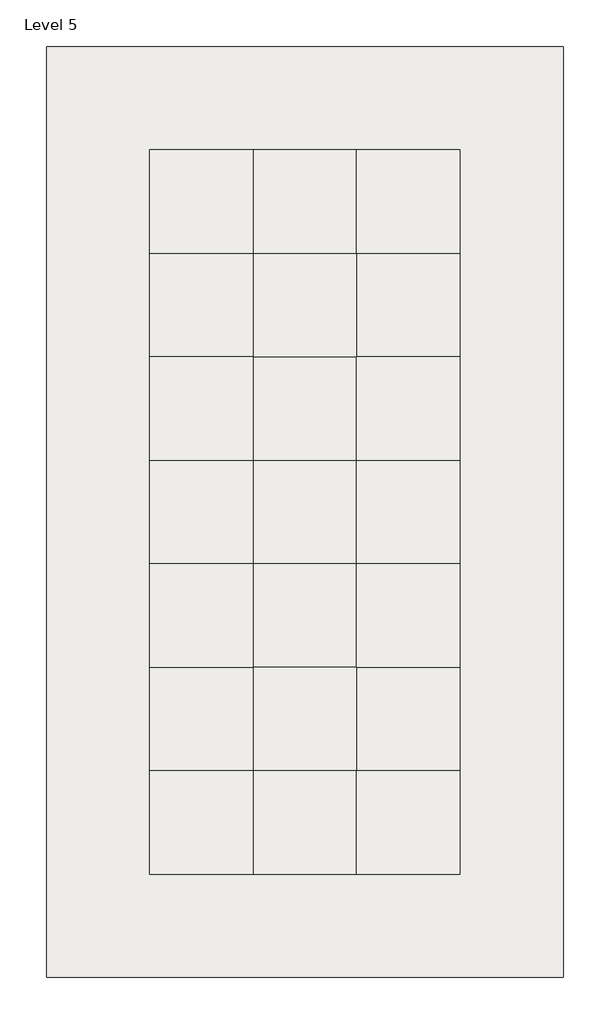
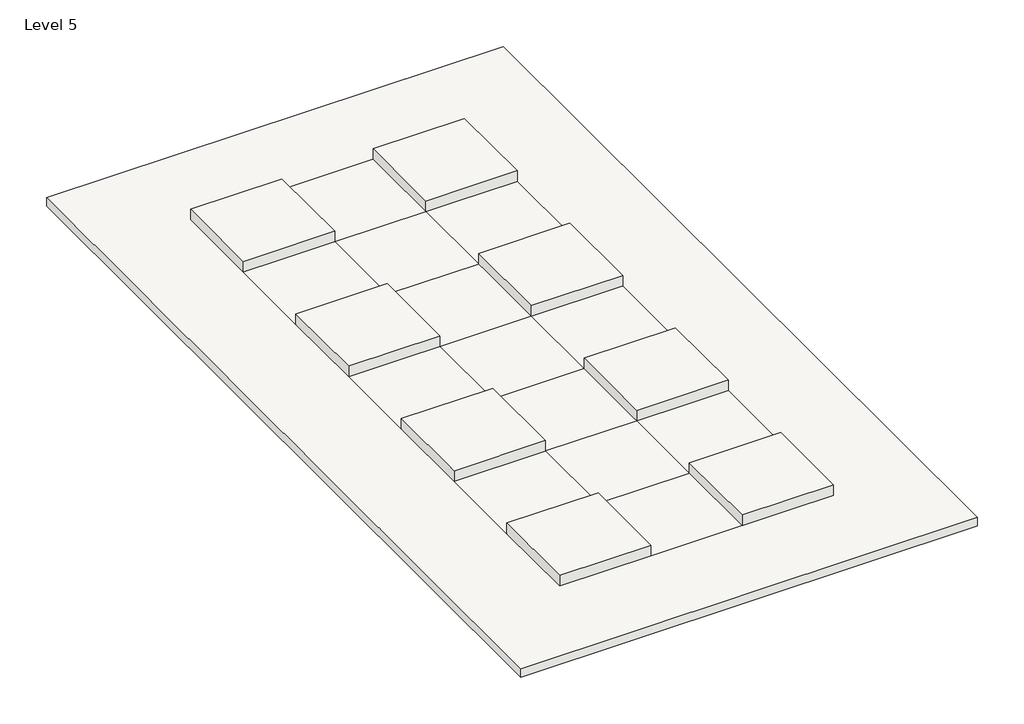
# One storey: 9 roofs.
"""IFC4 building model written with IfcOpenShell, lengths in millimetres."""

from ifc_helpers import new_model, si_unit, origin, place, context, project, spatial, faceted_brep, element, save

model = new_model("IFC4")

# Units and contexts
model_context = context("Model", 3, world=origin())
ifc_project = project(units=[si_unit("LENGTHUNIT", "METRE", prefix="MILLI")], contexts=[model_context])

# Site, building, storey
site = spatial("IfcSite", under=ifc_project)
building = spatial("IfcBuilding", under=site)
storey = spatial("IfcBuildingStorey", under=building, Name="Level 5", Elevation=20000.0)

# Roofs
placement = place(None, origin())
element("IfcRoof", 1, ObjectType="Bauder_RoofCoveringSystem_ExtensiveGreenRoofSystem_WildflowerBlanket", at=placement, inside=storey, context=model_context, shape_type="Brep", body=[
    faceted_brep([(-674.7340554, 1676.2074539, 20000.0), (1325.2659446, 1676.2074539, 20000.0), (1325.2659446, -323.7925461, 20000.0), (-674.7340554, -323.7925461, 20000.0), (1325.2659446, 1676.2074539, 20445.0), (-674.7340554, 1676.2074539, 20445.0), (-674.7340554, -323.7925461, 20445.0), (1325.2659446, -323.7925461, 20445.0), (1325.2659446, 1676.2074539, 20200.0), (-674.7340554, 1676.2074539, 20200.0), (-674.7340554, -323.7925461, 20200.0), (1325.2659446, -323.7925461, 20200.0)], [[[0, 1, 2, 3]], [[4, 5, 6, 7]], [[5, 4, 8, 1, 0, 9]], [[6, 5, 9, 0, 3, 10]], [[7, 6, 10, 3, 2, 11]], [[4, 7, 11, 2, 1, 8]]]),
])
element("IfcRoof", 2, ObjectType="Bauder_RoofCoveringSystem_ExtensiveGreenRoofSystem_WildflowerBlanket", at=placement, inside=storey, context=model_context, shape_type="Brep", body=[
    faceted_brep([(3325.2659446, 1676.2074539, 20000.0), (5325.2659446, 1676.2074539, 20000.0), (5325.2659446, -323.7925461, 20000.0), (3325.2659446, -323.7925461, 20000.0), (5325.2659446, 1676.2074539, 20445.0), (3325.2659446, 1676.2074539, 20445.0), (3325.2659446, -323.7925461, 20445.0), (5325.2659446, -323.7925461, 20445.0), (5325.2659446, 1676.2074539, 20200.0), (3325.2659446, 1676.2074539, 20200.0), (3325.2659446, -323.7925461, 20200.0), (5325.2659446, -323.7925461, 20200.0)], [[[0, 1, 2, 3]], [[4, 5, 6, 7]], [[5, 4, 8, 1, 0, 9]], [[6, 5, 9, 0, 3, 10]], [[7, 6, 10, 3, 2, 11]], [[4, 7, 11, 2, 1, 8]]]),
])
element("IfcRoof", 3, ObjectType="Bauder_RoofCoveringSystem_ExtensiveGreenRoofSystem_WildflowerBlanket", at=placement, inside=storey, context=model_context, shape_type="Brep", body=[
    faceted_brep([(3325.2659446, -2323.7925461, 20000.0), (5325.2659446, -2323.7925461, 20000.0), (5325.2659446, -4323.7925461, 20000.0), (3325.2659446, -4323.7925461, 20000.0), (5325.2659446, -2323.7925461, 20445.0), (3325.2659446, -2323.7925461, 20445.0), (3325.2659446, -4323.7925461, 20445.0), (5325.2659446, -4323.7925461, 20445.0), (5325.2659446, -2323.7925461, 20200.0), (3325.2659446, -2323.7925461, 20200.0), (3325.2659446, -4323.7925461, 20200.0), (5325.2659446, -4323.7925461, 20200.0)], [[[0, 1, 2, 3]], [[4, 5, 6, 7]], [[5, 4, 8, 1, 0, 9]], [[6, 5, 9, 0, 3, 10]], [[7, 6, 10, 3, 2, 11]], [[4, 7, 11, 2, 1, 8]]]),
])
element("IfcRoof", 4, ObjectType="Bauder_RoofCoveringSystem_ExtensiveGreenRoofSystem_WildflowerBlanket", at=placement, inside=storey, context=model_context, shape_type="Brep", body=[
    faceted_brep([(3325.2659446, -6323.7925461, 20000.0), (5325.2659446, -6323.7925461, 20000.0), (5325.2659446, -8323.7925461, 20000.0), (3325.2659446, -8323.7925461, 20000.0), (5325.2659446, -6323.7925461, 20445.0), (3325.2659446, -6323.7925461, 20445.0), (3325.2659446, -8323.7925461, 20445.0), (5325.2659446, -8323.7925461, 20445.0), (3325.2659446, -6323.7925461, 20200.0), (5325.2659446, -6323.7925461, 20200.0), (3325.2659446, -8323.7925461, 20200.0), (5325.2659446, -8323.7925461, 20200.0)], [[[0, 1, 2, 3]], [[4, 5, 6, 7]], [[0, 8, 5, 4, 9, 1]], [[3, 10, 6, 5, 8, 0]], [[2, 11, 7, 6, 10, 3]], [[1, 9, 4, 7, 11, 2]]]),
])
element("IfcRoof", 5, ObjectType="Bauder_RoofCoveringSystem_ExtensiveGreenRoofSystem_WildflowerBlanket", at=placement, inside=storey, context=model_context, shape_type="Brep", body=[
    faceted_brep([(3325.2659446, -10323.7925461, 20000.0), (5325.2659446, -10323.7925461, 20000.0), (5325.2659446, -12323.7925461, 20000.0), (3325.2659446, -12323.7925461, 20000.0), (5325.2659446, -10323.7925461, 20445.0), (3325.2659446, -10323.7925461, 20445.0), (3325.2659446, -12323.7925461, 20445.0), (5325.2659446, -12323.7925461, 20445.0), (3325.2659446, -10323.7925461, 20200.0), (5325.2659446, -10323.7925461, 20200.0), (3325.2659446, -12323.7925461, 20200.0), (5325.2659446, -12323.7925461, 20200.0)], [[[0, 1, 2, 3]], [[4, 5, 6, 7]], [[0, 8, 5, 4, 9, 1]], [[3, 10, 6, 5, 8, 0]], [[2, 11, 7, 6, 10, 3]], [[1, 9, 4, 7, 11, 2]]]),
])
element("IfcRoof", 6, ObjectType="Bauder_RoofCoveringSystem_ExtensiveGreenRoofSystem_WildflowerBlanket", at=placement, inside=storey, context=model_context, shape_type="Brep", body=[
    faceted_brep([(-674.7340554, -10323.7925461, 20000.0), (1325.2659446, -10323.7925461, 20000.0), (1325.2659446, -12323.7925461, 20000.0), (-674.7340554, -12323.7925461, 20000.0), (1325.2659446, -10323.7925461, 20445.0), (-674.7340554, -10323.7925461, 20445.0), (-674.7340554, -12323.7925461, 20445.0), (1325.2659446, -12323.7925461, 20445.0), (1325.2659446, -10323.7925461, 20200.0), (-674.7340554, -10323.7925461, 20200.0), (-674.7340554, -12323.7925461, 20200.0), (1325.2659446, -12323.7925461, 20200.0)], [[[0, 1, 2, 3]], [[4, 5, 6, 7]], [[5, 4, 8, 1, 0, 9]], [[6, 5, 9, 0, 3, 10]], [[7, 6, 10, 3, 2, 11]], [[4, 7, 11, 2, 1, 8]]]),
])
element("IfcRoof", 7, ObjectType="Bauder_RoofCoveringSystem_ExtensiveGreenRoofSystem_WildflowerBlanket", at=placement, inside=storey, context=model_context, shape_type="Brep", body=[
    faceted_brep([(-674.7340554, -6323.7925461, 20000.0), (1325.2659446, -6323.7925461, 20000.0), (1325.2659446, -8323.7925461, 20000.0), (-674.7340554, -8323.7925461, 20000.0), (1325.2659446, -6323.7925461, 20445.0), (-674.7340554, -6323.7925461, 20445.0), (-674.7340554, -8323.7925461, 20445.0), (1325.2659446, -8323.7925461, 20445.0), (1325.2659446, -6323.7925461, 20200.0), (-674.7340554, -6323.7925461, 20200.0), (-674.7340554, -8323.7925461, 20200.0), (1325.2659446, -8323.7925461, 20200.0)], [[[0, 1, 2, 3]], [[4, 5, 6, 7]], [[5, 4, 8, 1, 0, 9]], [[6, 5, 9, 0, 3, 10]], [[7, 6, 10, 3, 2, 11]], [[4, 7, 11, 2, 1, 8]]]),
])
element("IfcRoof", 8, ObjectType="Bauder_RoofCoveringSystem_ExtensiveGreenRoofSystem_WildflowerBlanket", at=placement, inside=storey, context=model_context, shape_type="Brep", body=[
    faceted_brep([(-674.7340554, -2323.7925461, 20000.0), (1325.2659446, -2323.7925461, 20000.0), (1325.2659446, -4323.7925461, 20000.0), (-674.7340554, -4323.7925461, 20000.0), (1325.2659446, -2323.7925461, 20445.0), (-674.7340554, -2323.7925461, 20445.0), (-674.7340554, -4323.7925461, 20445.0), (1325.2659446, -4323.7925461, 20445.0), (1325.2659446, -2323.7925461, 20200.0), (-674.7340554, -2323.7925461, 20200.0), (-674.7340554, -4323.7925461, 20200.0), (1325.2659446, -4323.7925461, 20200.0)], [[[0, 1, 2, 3]], [[4, 5, 6, 7]], [[5, 4, 8, 1, 0, 9]], [[6, 5, 9, 0, 3, 10]], [[7, 6, 10, 3, 2, 11]], [[4, 7, 11, 2, 1, 8]]]),
])
element("IfcRoof", 9, ObjectType="Roof_Concrete-200mm", at=placement, inside=storey, context=model_context, shape_type="Brep", body=[
    faceted_brep([(-2674.7340554, -14323.7925461, 20200.0), (-2674.7340554, -14323.7925461, 20000.0), (7325.2659446, -14323.7925461, 20000.0), (7325.2659446, -14323.7925461, 20200.0), (-2674.7340554, 3676.2074539, 20200.0), (-2674.7340554, 3676.2074539, 20000.0), (7325.2659446, 3676.2074539, 20200.0), (7325.2659446, 3676.2074539, 20000.0), (3325.2659446, 1676.2074539, 20200.0), (1325.2659446, 1676.2074539, 20200.0), (1325.2659446, -323.7925461, 20200.0), (3325.2659446, -323.7925461, 20200.0), (1325.2659446, 1676.2074539, 20000.0), (3325.2659446, 1676.2074539, 20000.0), (3325.2659446, -323.7925461, 20000.0), (1325.2659446, -323.7925461, 20000.0), (1325.2659446, -2323.7925461, 20200.0), (-674.7340554, -323.7925461, 20200.0), (-674.7340554, -2323.7925461, 20200.0), (3325.2659446, -2323.7925461, 20200.0), (5325.2659446, -2323.7925461, 20200.0), (5325.2659446, -323.7925461, 20200.0), (-674.7340554, -2323.7925461, 20000.0), (-674.7340554, -323.7925461, 20000.0), (1325.2659446, -2323.7925461, 20000.0), (3325.2659446, -2323.7925461, 20000.0), (5325.2659446, -323.7925461, 20000.0), (5325.2659446, -2323.7925461, 20000.0), (1325.2659446, -4323.7925461, 20200.0), (3325.2659446, -4323.7925461, 20200.0), (3325.2659446, -4323.7925461, 20000.0), (1325.2659446, -4323.7925461, 20000.0), (1325.2659446, -6323.7925461, 20200.0), (-674.7340554, -4323.7925461, 20200.0), (-674.7340554, -6323.7925461, 20200.0), (5325.2659446, -6323.7925461, 20200.0), (5325.2659446, -4323.7925461, 20200.0), (3325.2659446, -6323.7925461, 20200.0), (-674.7340554, -6323.7925461, 20000.0), (-674.7340554, -4323.7925461, 20000.0), (1325.2659446, -6323.7925461, 20000.0), (3325.2659446, -6323.7925461, 20000.0), (5325.2659446, -4323.7925461, 20000.0), (5325.2659446, -6323.7925461, 20000.0), (1325.2659446, -12323.7925461, 20200.0), (3325.2659446, -12323.7925461, 20200.0), (3325.2659446, -10323.7925461, 20200.0), (1325.2659446, -10323.7925461, 20200.0), (3325.2659446, -12323.7925461, 20000.0), (1325.2659446, -12323.7925461, 20000.0), (1325.2659446, -10323.7925461, 20000.0), (3325.2659446, -10323.7925461, 20000.0), (1325.2659446, -8323.7925461, 20200.0), (-674.7340554, -8323.7925461, 20200.0), (-674.7340554, -10323.7925461, 20200.0), (3325.2659446, -8323.7925461, 20200.0), (5325.2659446, -10323.7925461, 20200.0), (5325.2659446, -8323.7925461, 20200.0), (-674.7340554, -10323.7925461, 20000.0), (-674.7340554, -8323.7925461, 20000.0), (1325.2659446, -8323.7925461, 20000.0), (3325.2659446, -8323.7925461, 20000.0), (5325.2659446, -8323.7925461, 20000.0), (5325.2659446, -10323.7925461, 20000.0), (-674.7340554, 1676.2074539, 20000.0), (-674.7340554, 1676.2074539, 20200.0), (5325.2659446, 1676.2074539, 20200.0), (5325.2659446, 1676.2074539, 20000.0), (5325.2659446, -12323.7925461, 20000.0), (5325.2659446, -12323.7925461, 20200.0), (-674.7340554, -12323.7925461, 20000.0), (-674.7340554, -12323.7925461, 20200.0)], [[[0, 1, 2, 3]], [[1, 0, 4, 5]], [[6, 7, 5, 4]], [[3, 2, 7, 6]], [[8, 9, 10, 11]], [[12, 13, 14, 15]], [[16, 10, 17, 18]], [[11, 10, 16, 19]], [[20, 21, 11, 19]], [[22, 23, 15, 24]], [[15, 14, 25, 24]], [[25, 14, 26, 27]], [[19, 16, 28, 29]], [[24, 25, 30, 31]], [[32, 28, 33, 34]], [[35, 36, 29, 37]], [[38, 39, 31, 40]], [[41, 30, 42, 43]], [[44, 45, 46, 47]], [[48, 49, 50, 51]], [[47, 52, 53, 54]], [[47, 46, 55, 52]], [[56, 57, 55, 46]], [[58, 59, 60, 50]], [[51, 50, 60, 61]], [[51, 61, 62, 63]], [[52, 55, 37, 32]], [[29, 28, 32, 37]], [[61, 60, 40, 41]], [[31, 30, 41, 40]], [[9, 12, 15, 10]], [[10, 15, 23, 17]], [[17, 23, 64, 65]], [[12, 9, 65, 64]], [[66, 67, 26, 21]], [[21, 26, 14, 11]], [[11, 14, 13, 8]], [[67, 66, 8, 13]], [[20, 27, 42, 36]], [[36, 42, 30, 29]], [[29, 30, 25, 19]], [[27, 20, 19, 25]], [[16, 24, 31, 28]], [[28, 31, 39, 33]], [[33, 39, 22, 18]], [[24, 16, 18, 22]], [[32, 40, 60, 52]], [[52, 60, 59, 53]], [[53, 59, 38, 34]], [[40, 32, 34, 38]], [[35, 43, 62, 57]], [[57, 62, 61, 55]], [[55, 61, 41, 37]], [[43, 35, 37, 41]], [[56, 63, 68, 69]], [[69, 68, 48, 45]], [[45, 48, 51, 46]], [[63, 56, 46, 51]], [[47, 50, 49, 44]], [[44, 49, 70, 71]], [[71, 70, 58, 54]], [[50, 47, 54, 58]], [[4, 0, 3, 6], [9, 8, 66, 21, 20, 36, 35, 57, 56, 69, 45, 44, 71, 54, 53, 34, 33, 18, 17, 65]], [[7, 2, 1, 5], [13, 12, 64, 23, 22, 39, 38, 59, 58, 70, 49, 48, 68, 63, 62, 43, 42, 27, 26, 67]]]),
])

save(model, "model.ifc")

# Revit data of these elements
# Type "Bauder_RoofCoveringSystem_ExtensiveGreenRoofSystem_WildflowerBlanket"
#   Keynote = "Q37"
#   Type IFC Predefined Type = "FLAT_ROOF"
#   Export Type to IFC As = "IfcRoofType"
#   Model = "Bauder Biodiverse Wildflower Blanket - Extensive Green Roof System"
#   Manufacturer = "Bauder Ltd"
#   Type Comments = "Wildflower Blanket"
#   URL = "https://www.bauder.co.uk/"
#   Description = "Bauder Biodiverse GreenRoof system incorporating WB 25 mm UK Native Species Wildflower Blanket with Biodiverse Substrate, Filter Fleece, DSE40 Polyethylene Drainage and Protection Layer, and FSM600 Polyester-Polypropylene fibre protection mat."
#   Assembly Code = "B3010"
#   NBSDescription = "Extensive green roof system"
#   NBSReference = "45-40-47/130"
#   BIMObjectName = "Bauder_RoofCoveringSystem_ExtensiveGreenRoofSystem_WildflowerBlanket"
#   AccessibilityPerformance = "n/a"
#   CodePerformance = "n/a"
#   Color = "n/a"
#   Constituents = "n/a"
#   DurationUnit = "Year"
#   ExpectedLife = "n/a"
#   Features = "This BIM Object must be supported by a project specific specification from Bauder, incorporating system build-up, detail design and performance calculations if a full Bauder system guarantee is required. Please contact your local Bauder Representative or technical@bauder.co.uk"
#   Finish = "n/a"
#   Grade = "n/a"
#   Material = "n/a"
#   ModelReference = "Bauder Biodiverse Wildflower Blanket - Extensive Green Roof System"
#   Name = "RoofCoveringSystem_Bauder_ExtensiveGreenRoofSystem"
#   ReplacementCost = "n/a"
#   Shape = "n/a"
#   Size = "n/a"
#   SustainabilityPerformance = "Bauder Germany ISO14001: Certificate No.: 70499/03-15 e, Bauder UK ISO14001:Certificate No. 19ACM6595R, EN1271, BREEAM Credits Available"
#   WarrantyDescription = "Guarantee options could include ‘Product’, ‘Product and Workmanship’ and ‘Product, Workmanship and Design’ Guarantees. All guarantees available for this system are subject to the works being carried out in accordance with the Bauder specification and being installed by a Bauder Approved installer. For full details and further information regarding guarantees and alternative systems please contact your local Bauder Representative or technical@bauder.co.uk"
#   WarrantyDurationLabor = "n/a"
#   WarrantyDurationParts = "n/a"
#   WarrantyDurationUnit = "Year"
#   WarrantyGuarantorLabor = "n/a"
#   WarrantyGuarantorParts = "technical@bauder.co.uk"
#   Certification = "Comply with GRO Green Roof Code of Practice and FLL Standards"
#   EdgeRestraints = "Perforated edge trim where required, refer to Bauder Project Specific Specification"
#   MoistureControlDrainageAncillaries = "n/a"
#   MoistureControlDrainageLayer = "Bauder DSE40 40 mm Polyethylene Drainage and Protection Layer"
#   MoistureControlFilterMembrane = "Bauder Filter Fleece 1 mm Polypropylene Filter Fleece"
#   MoistureControlMoistureRetentionMat = "Polypropylene mesh bonded to a moisture permeable base carrier sheet integral to the Blanket"
#   PlantingSystemsAntierosionMat = "Jute Net where exposed, refer to Bauder Project Specific Specification"
#   PlantingSystemsPlantingMedium = "Bauder Biodiverse Substrate Recycled crushed brick, expanded clay shale and composted pine bark"
#   PlantingSystemsVegetation = "Bauder WB 25 mm UK Native Species Wildflower Blanket"
#   PlantingSystemsVegetationBarrier = "20-40 mm Rounded-Washed Stones, refer to Bauder Project Specific Specification"
#   ProjectSpecificationAndDesign = "This BIM Object must be supported by a project specific specification from Bauder, incorporating system build-up, detail design and performance calculations if a full Bauder system warranty is required. Please contact your local Bauder Representative or technical@bauder.co.uk"
#   ProtectionProtectionLayer = "Bauder FSM600 4 mm Polyester-Polypropylene fibre protection mat"
#   ProtectionRootBarrier = "As per project specific Bauder Specification"
#   ProtectionSeparationLayer = "n/a"
#   SystemManufacturer = "Bauder Ltd"
#   WarrantyConsiderations = "All guarantees available for this system are subject to the works being carried out in accordance with the Bauder specification and being installed by a Bauder Approved installer. For full details and further information regarding guarantees and alternative systems please contact your local Bauder Representative or technical@bauder.co.uk"
#   Update = "1900-12-31T23:59:59"
#   Documentation = "https://www.bauder.co.uk/technical-centre/technical-literature/system-brochures"
#   DocumentReference = "http://www.bauder.co.uk/"
#   IfcExportAs = "IfcRoofType"
#   IfcExportType = "FLAT_ROOF"
#   MethodOfMesurement = "n/a"
#   Process = "Replacement at service life intervals"
#   FireRating = "n/a"
#   _Author = "AM"
#   _AuthorizedBy = "bimstore"
#   _CreatedBy = "technical@bauder.co.uk"
#   _DistributedBy = "www.bimstore.co"
#   AssetType = "Fixed"
#   ClassificationName = "Uniclass2015"
#   ClassificationValue = "Ss_45_40_47_09"
#   CreatedBy = "technical@bauder.co.uk"
#   CreatedOn = "2023-02-10 T00:00:00"
#   DocumentationCertificates = "n/a"
#   DocumentationInstallationGuide = "https://www.bauder.co.uk/technical-centre"
#   DocumentationLiterature = "https://www.bauder.co.uk/technical-centre"
#   DocumentationMaintenance = "https://www.bauder.co.uk/technical-centre/maintenance-advice"
#   DocumentationTechnical = "https://www.bauder.co.uk/green-roofs/extensive-green-roofs/biodiverse-or-brown-roofs/wildflower-blanket"
#   ManufacturerName = "Bauder Ltd"
#   ModelNumber = "0905_WB-BioS-FF-D4-F6"
#   ProductionYear = "2017"
#   ReferencedStandard = "n/a"
#   SpareParts = "n/a"
#   TypeName = "Wildflower Blanket"
#   NBSNote = "n/a"
#   NBSObjectName = "Bauder - Extensive green roof system"
#   NBSOfficeMasterTag = "n/a"
#   Ballast = "n/a"
#   CarrierMembraneFixing = "n/a"
#   CarrierMembraneType = "n/a"
#   FillToPerimeterUpstands = "n/a"
#   FilterLayer = "n/a"
#   InsulationFixing = "n/a"
#   InsulationType = "n/a"
#   LiquidAppliedWaterproofCoatingReinforcement = "n/a"
#   LiquidAppliedWaterproofCoatingSurfaceTreatment = "n/a"
#   LiquidAppliedWaterproofCoatingType = "n/a"
#   PreparationExistingSubstrates = "n/a"
#   PreparationHorizontalWork = "n/a"
#   PreparationSkirtingsAndVerticalWork = "n/a"
#   ProtectionLayer = "n/a"
#   SystemAccessories = "n/a"
#   WaterproofCoveringFirstLayerAttachment = "n/a"
#   WaterproofCoveringFirstLayerType = "n/a"
#   WaterproofCoveringIntermediateLayerAttachment = "n/a"
#   WaterproofCoveringIntermediateLayerType = "n/a"
#   WaterproofCoveringTopLayerAttachment = "n/a"
#   InsulationAttachment = "n/a"
#   IsolatingLayer = "n/a"
#   CarrierMembraneAttachment = "n/a"
#   LiquidAppliedWaterproofCoatingWearingCourse = "n/a"
#   VapourControlLayer = "n/a"
#   VapourControlLayerAttachment_Bauder = "n/a"
#   WaterproofCoveringJoints = "n/a"
#   WaterproofCoveringType = "n/a"
#   SeparatingLayer = "n/a"
#   WaterproofCoveringAccessories = "Yes"
#   WaterproofCoveringAttachment = "n/a"
#   UpperProtectionLayer = "n/a"
#   LowerProtectionLayer = "n/a"
#   WaterproofCoveringTopLayerType = "n/a"
#   DetailWorkAncillaryItems = "Detail as per project specific Bauder Specification"
#   DetailWorkCoverStrips = "Detail as per project specific Bauder Specification"
#   DetailWorkFlashings = "Detail as per project specific Bauder Specification"
#   DetailWorkSkirtingsAndUpstands = "Detail as per project specific Bauder Specification"
#   DetailWorkWeltedDrips = "Detail as per project specific Bauder Specification"
#   OverlayFixing = "n/a"
#   OverlayType = "n/a"
#   SurfaceProtection = "n/a"
#   VapourControlLayerAttachment = "n/a"
#   VapourControlLayerType = "n/a"
#   Cost = 0
#   NominalHeight = 0 mm
#   NominalLength = 0 mm
#   TotalArea = 0 m²
#   NominalDepth = 0 mm
#   IsExternal = yes
#   _BimSpecGuid = 0
#   _BSBibleVersion = 16
#   _CurrentRevision = 4
#   Layers, outside or top first: 100 mm "Bauder_Vegetation_BauderGREEN-WB-Wildflower-Blanket" (function 5); 100 mm "Bauder_ExtensiveSubstrate_BauderGREEN-SUB-BM-UK" (function 2); 1 mm "Bauder_FilterFleece_BauderGREEN-FV-125-100" (function 3); 40 mm "Bauder_DrainageBoard_BauderGREEN-DSE-40" (function 3); 4 mm "Bauder_ProtectionMat_BauderGREEN-FSM-600" (function 3); 200 mm "Concrete" (function 1)
# Type "Roof_Concrete-200mm"
#   Layers, outside or top first: 200 mm "Concrete" (function 1)
# Elements 1, 2, 3, 4, 5, 6, 7, 8 (IfcRoof, "Bauder_RoofCoveringSystem_ExtensiveGreenRoofSystem_WildflowerBlanket")
#   built-in parameter 1001705 = 67.0768 (stored number, unit not read)
#   built-in parameter 1001710 = 33615
#   Phase Created = New Construction
#   Materials on its faces: "Concrete", "Bauder_Vegetation_BauderGREEN-WB-Wildflower-Blanket"
# Element 9 (IfcRoof, "Roof_Concrete-200mm")
#   built-in parameter 1001710 = 33615
#   Phase Created = New Construction
#   Materials on its faces: "Concrete"
# Materials
#   "Bauder_Vegetation_BauderGREEN-WB-Wildflower-Blanket": class "Unassigned", colour RGB 71 83 38, transparency 0, Mtrl_Author = "AM", Mtrl_AuthorizedBy = "bimstore", Mtrl_DistributedBy = "www.bimstore.co", Mtrl_AccessibilityPerformance = "n/a", Mtrl_AssetIdentifier = "Please record on commissioning", Mtrl_AssetType = "Fixed", Mtrl_BarCode = "Please record on commissioning", Mtrl_ClassificationName = "Uniclass2020", Mtrl_ClassificationValue = "Ss_45_40_47_09", Mtrl_CodePerformance = "n/a", Mtrl_Color = "n/a", Mtrl_Constituents = "n/a", Mtrl_CreatedBy = "technical@bauder.co.uk", Mtrl_CreatedOn = "2023-02-10 T00:00:00", Mtrl_DocumentationCertificates = "https://www.bimstore.co/products/extensive-green-roof-system-wildflower-blanket/document/product-certificates", Mtrl_DocumentationInstallationGuide = "https://www.bimstore.co/products/extensive-green-roof-system-wildflower-blanket/document/installation-guide", Mtrl_DocumentationLiterature = "https://www.bimstore.co/products/extensive-green-roof-system-wildflower-blanket/document/product-literature", Mtrl_DocumentationMaintenance = "https://www.bimstore.co/products/extensive-green-roof-system-wildflower-blanket/document/maintenance-information", Mtrl_DocumentationTechnical = "https://www.bimstore.co/products/extensive-green-roof-system-wildflower-blanket/document/technical-data-sheet", Mtrl_DurationUnit = "Year", Mtrl_Features = "n/a", Mtrl_Finish = "n/a", Mtrl_Grade = "n/a", Mtrl_InstallationDate = "Please record on commissioning", Mtrl_ManufacturerName = "Bauder Ltd", Mtrl_Material = "Substrate and wildflower plants, embedded in a nylon mesh, with a moisture retention fleece", Mtrl_ModelNumber = "BauderGREEN-WB-Wildflower-Blanket", Mtrl_ModelReference = "Vegetation", Mtrl_ProductionYear = "2023", Mtrl_ReferencedStandard = "n/a", Mtrl_Shape = "n/a", Mtrl_Size = "n/a", Mtrl_SpareParts = "n/a", Mtrl_TypeName = "BauderGREEN-WB-Wildflower-Blanket", Mtrl_WarrantyDescription = "As part of Bauder system guarantee, per specification", Mtrl_WarrantyDurationUnit = "Year", Mtrl_WarrantyGuarantorLabor = "technical@bauder.co.uk", Mtrl_WarrantyGuarantorParts = "technical@bauder.co.uk", Mtrl_WarrantyStartDate = "Please record on commissioning", Mtrl_IfcExportAs = "IfcRoofType", Mtrl_IfcExportType = "FLAT_ROOF", Mtrl_BIMObjectName = "Bauder_Vegetation_BauderGREEN-WB-Wildflower-Blanket", Mtrl_NBSDescription = "n/a", Mtrl_NBSNote = "n/a", Mtrl_NBSObjectName = "n/a", Mtrl_NBSOfficeMasterTag = "n/a", Mtrl_NBSReference = "Q37", Mtrl_Ballast = "n/a", Mtrl_CarrierMembraneAttachment = "n/a", Mtrl_CarrierMembraneFixing = "n/a", Mtrl_CarrierMembraneType = "n/a", Mtrl_Certification = "Comply with GRO Green Roof Code of Practice and FLL Standards", Mtrl_DetailWorkAncillaryItems = "Detail as per project specific Bauder Specification", Mtrl_DetailWorkCoverStrips = "Detail as per project specific Bauder Specification", Mtrl_DetailWorkFlashings = "Detail as per project specific Bauder Specification", Mtrl_DetailWorkSkirtingsAndUpstands = "Detail as per project specific Bauder Specification", Mtrl_DetailWorkWeltedDrips = "Detail as per project specific Bauder Specification", Mtrl_EdgeRestraints = "Detail as per project specific Bauder Specification", Mtrl_FillToPerimeterUpstands = "n/a", Mtrl_FilterLayer = "n/a", Mtrl_InsulationAttachment = "As per project specific Bauder Specification", Mtrl_InsulationFixing = "As per project specific Bauder Specification", Mtrl_InsulationType = "As per project specific Bauder Specification", Mtrl_IsolatingLayer = "n/a", Mtrl_LiquidAppliedWaterproofCoatingReinforcement = "As per project specific Bauder Specification", Mtrl_LiquidAppliedWaterproofCoatingSurfaceTreatment = "As per project specific Bauder Specification", Mtrl_LiquidAppliedWaterproofCoatingType = "As per project specific Bauder Specification", Mtrl_LiquidAppliedWaterproofCoatingWearingCourse = "As per project specific Bauder Specification", Mtrl_LowerProtectionLayer = "n/a", Mtrl_MoistureControlDrainageAncillaries = "n/a", Mtrl_MoistureControlDrainageLayer = "n/a", Mtrl_MoistureControlFilterMembrane = "n/a", Mtrl_MoistureControlMoistureRetentionMat = "n/a", Mtrl_OverlayFixing = "n/a", Mtrl_OverlayType = "n/a", Mtrl_PlantingSystemsAntierosionMat = "n/a", Mtrl_PlantingSystemsPlantingMedium = "As per project specific Bauder Specification", Mtrl_PlantingSystemsVegetation = "As per project specific Bauder Specification", Mtrl_PlantingSystemsVegetationBarrier = "As per project specific Bauder Specification", Mtrl_PreparationExistingSubstrates = "n/a", Mtrl_PreparationHorizontalWork = "n/a", Mtrl_PreparationSkirtingsAndVerticalWork = "n/a", Mtrl_ProjectSpecificationAndDesign = "This BIM Object must be supported by a project specific specification from Bauder, incorporating system build-up, detail design and performance calculations if a full Bauder system warranty is required. Please contact your local Bauder Representative or technical@bauder.co.uk", Mtrl_ProtectionLayer = "n/a", Mtrl_ProtectionProtectionLayer = "n/a", Mtrl_ProtectionRootBarrier = "As per project specific Bauder Specification", Mtrl_ProtectionSeparationLayer = "n/a", Mtrl_SeparatingLayer = "n/a", Mtrl_SurfaceProtection = "n/a", Mtrl_SystemAccessories = "n/a", Mtrl_SystemManufacturer = "Bauder Ltd", Mtrl_Update = "1900-12-31 T23:59:59", Mtrl_UpperProtectionLayer = "n/a", Mtrl_VapourControlLayerAttachment = "As per project specific Bauder Specification", Mtrl_VapourControlLayerAttachment_Bauder = "As per project specific Bauder Specification", Mtrl_VapourControlLayerType = "As per project specific Bauder Specification", Mtrl_WarrantyConsiderations = "All guarantees available for this system are subject to the works being carried out in accordance with the Bauder specification and being installed by a Bauder Approved installer. For full details and further information regarding guarantees and alternative systems please contact your local Bauder Representative or technical@bauder.co.uk", Mtrl_WaterproofCoveringAccessories = "As per project specific Bauder Specification", Mtrl_WaterproofCoveringAttachment = "As per project specific Bauder Specification", Mtrl_WaterproofCoveringFirstLayerAttachment = "As per project specific Bauder Specification", Mtrl_WaterproofCoveringFirstLayerType = "As per project specific Bauder Specification", Mtrl_WaterproofCoveringIntermediateLayerAttachment = "As per project specific Bauder Specification", Mtrl_WaterproofCoveringIntermediateLayerType = "As per project specific Bauder Specification", Mtrl_WaterproofCoveringJoints = "As per project specific Bauder Specification", Mtrl_WaterproofCoveringTopLayerAttachment = "As per project specific Bauder Specification", Mtrl_WaterproofCoveringTopLayerType = "As per project specific Bauder Specification", Mtrl_WaterproofCoveringType = "As per project specific Bauder Specification", Cost = 0, Mtrl_ReplacementCost = 0, Mtrl_NominalDepth = 30 mm, Mtrl_NominalHeight = 0 mm, Mtrl_NominalLength = 0 mm, Mtrl_BimSpecGuid = 0, Mtrl_BSBibleVersion = 17, Mtrl_CurrentRevision = 2, Mtrl_ExpectedLife = 0, Mtrl_SerialNumber = 0, Mtrl_WarrantyDurationLabor = 0, Mtrl_WarrantyDurationParts = 0
#   "Bauder_ExtensiveSubstrate_BauderGREEN-SUB-BM-UK": class "Unassigned", colour RGB 255 255 255, transparency 0, Mtrl_Author = "AM", Mtrl_AuthorizedBy = "bimstore", Mtrl_DistributedBy = "www.bimstore.co", Mtrl_AccessibilityPerformance = "n/a", Mtrl_AssetIdentifier = "Please record on commissioning", Mtrl_AssetType = "Fixed", Mtrl_BarCode = "Please record on commissioning", Mtrl_ClassificationName = "Uniclass2019", Mtrl_ClassificationValue = "n/a", Mtrl_CodePerformance = "n/a", Mtrl_Color = "n/a", Mtrl_Constituents = "n/a", Mtrl_CreatedBy = "technical@bauder.co.uk", Mtrl_CreatedOn = "2023-02-10 T00:00:00", Mtrl_DocumentationCertificates = "https://www.bimstore.co/products/extensive-green-roof-system-wildflower-blanket/document/product-certificates", Mtrl_DocumentationInstallationGuide = "https://www.bimstore.co/products/extensive-green-roof-system-wildflower-blanket/document/installation-guide", Mtrl_DocumentationLiterature = "https://www.bimstore.co/products/extensive-green-roof-system-wildflower-blanket/document/product-literature", Mtrl_DocumentationMaintenance = "https://www.bimstore.co/products/extensive-green-roof-system-wildflower-blanket/document/maintenance-information", Mtrl_DocumentationTechnical = "https://www.bimstore.co/products/extensive-green-roof-system-wildflower-blanket/document/technical-data-sheet", Mtrl_DurationUnit = "Year", Mtrl_Features = "n/a", Mtrl_Finish = "n/a", Mtrl_Grade = "n/a", Mtrl_InstallationDate = "Please record on commissioning", Mtrl_ManufacturerName = "Bauder Ltd", Mtrl_Material = "Recycled crushed brick, expanded clay, shale, composted pine bark", Mtrl_ModelNumber = "BauderGREEN-SUB-BM-UK", Mtrl_ModelReference = "Extensive Substrate", Mtrl_ProductionYear = "2023", Mtrl_ReferencedStandard = "n/a", Mtrl_Shape = "n/a", Mtrl_Size = "n/a", Mtrl_SpareParts = "n/a", Mtrl_TypeName = "BauderGREEN-SUB-BM-UK", Mtrl_WarrantyDescription = "As part of Bauder system guarantee, per specification", Mtrl_WarrantyDurationUnit = "Year", Mtrl_WarrantyGuarantorLabor = "technical@bauder.co.uk", Mtrl_WarrantyGuarantorParts = "technical@bauder.co.uk", Mtrl_WarrantyStartDate = "Please record on commissioning", Mtrl_IfcExportAs = "IfcRoofType", Mtrl_IfcExportType = "FLAT_ROOF", Mtrl_BIMObjectName = "Bauder_ExtensiveSubstrate_BauderGREEN-SUB-BM-UK", Mtrl_NBSDescription = "n/a", Mtrl_NBSNote = "n/a", Mtrl_NBSObjectName = "n/a", Mtrl_NBSOfficeMasterTag = "n/a", Mtrl_NBSReference = "Q37", Mtrl_Ballast = "n/a", Mtrl_CarrierMembraneAttachment = "n/a", Mtrl_CarrierMembraneFixing = "n/a", Mtrl_CarrierMembraneType = "n/a", Mtrl_Certification = "Comply with GRO Green Roof Code of Practice and FLL Standards", Mtrl_DetailWorkAncillaryItems = "Detail as per project specific Bauder Specification", Mtrl_DetailWorkCoverStrips = "Detail as per project specific Bauder Specification", Mtrl_DetailWorkFlashings = "Detail as per project specific Bauder Specification", Mtrl_DetailWorkSkirtingsAndUpstands = "Detail as per project specific Bauder Specification", Mtrl_DetailWorkWeltedDrips = "Detail as per project specific Bauder Specification", Mtrl_EdgeRestraints = "Detail as per project specific Bauder Specification", Mtrl_FillToPerimeterUpstands = "n/a", Mtrl_FilterLayer = "n/a", Mtrl_InsulationAttachment = "As per project specific Bauder Specification", Mtrl_InsulationFixing = "As per project specific Bauder Specification", Mtrl_InsulationType = "As per project specific Bauder Specification", Mtrl_IsolatingLayer = "n/a", Mtrl_LiquidAppliedWaterproofCoatingReinforcement = "As per project specific Bauder Specification", Mtrl_LiquidAppliedWaterproofCoatingSurfaceTreatment = "As per project specific Bauder Specification", Mtrl_LiquidAppliedWaterproofCoatingType = "As per project specific Bauder Specification", Mtrl_LiquidAppliedWaterproofCoatingWearingCourse = "As per project specific Bauder Specification", Mtrl_LowerProtectionLayer = "As per project specific Bauder Specification", Mtrl_MoistureControlDrainageAncillaries = "n/a", Mtrl_MoistureControlDrainageLayer = "n/a", Mtrl_MoistureControlFilterMembrane = "n/a", Mtrl_MoistureControlMoistureRetentionMat = "n/a", Mtrl_OverlayFixing = "n/a", Mtrl_OverlayType = "n/a", Mtrl_PlantingSystemsAntierosionMat = "n/a", Mtrl_PlantingSystemsPlantingMedium = "As per project specific Bauder Specification", Mtrl_PlantingSystemsVegetation = "As per project specific Bauder Specification", Mtrl_PlantingSystemsVegetationBarrier = "As per project specific Bauder Specification", Mtrl_PreparationExistingSubstrates = "n/a", Mtrl_PreparationHorizontalWork = "n/a", Mtrl_PreparationSkirtingsAndVerticalWork = "n/a", Mtrl_ProjectSpecificationAndDesign = "This BIM Object must be supported by a project specific specification from Bauder, incorporating system build-up, detail design and performance calculations if a full Bauder system warranty is required. Please contact your local Bauder Representative or technical@bauder.co.uk", Mtrl_ProtectionLayer = "n/a", Mtrl_ProtectionProtectionLayer = "n/a", Mtrl_ProtectionRootBarrier = "As per project specific Bauder Specification", Mtrl_ProtectionSeparationLayer = "n/a", Mtrl_SeparatingLayer = "n/a", Mtrl_SurfaceProtection = "n/a", Mtrl_SystemAccessories = "n/a", Mtrl_SystemManufacturer = "Bauder Ltd", Mtrl_Update = "1900-12-31 T23:59:59", Mtrl_UpperProtectionLayer = "n/a", Mtrl_VapourControlLayerAttachment = "As per project specific Bauder Specification", Mtrl_VapourControlLayerAttachment_Bauder = "As per project specific Bauder Specification", Mtrl_VapourControlLayerType = "As per project specific Bauder Specification", Mtrl_WarrantyConsiderations = "All guarantees available for this system are subject to the works being carried out in accordance with the Bauder specification and being installed by a Bauder Approved installer. For full details and further information regarding guarantees and alternative systems please contact your local Bauder Representative or technical@bauder.co.uk", Mtrl_WaterproofCoveringAccessories = "As per project specific Bauder Specification", Mtrl_WaterproofCoveringAttachment = "As per project specific Bauder Specification", Mtrl_WaterproofCoveringFirstLayerAttachment = "As per project specific Bauder Specification", Mtrl_WaterproofCoveringFirstLayerType = "As per project specific Bauder Specification", Mtrl_WaterproofCoveringIntermediateLayerAttachment = "As per project specific Bauder Specification", Mtrl_WaterproofCoveringIntermediateLayerType = "As per project specific Bauder Specification", Mtrl_WaterproofCoveringJoints = "As per project specific Bauder Specification", Mtrl_WaterproofCoveringTopLayerAttachment = "As per project specific Bauder Specification", Mtrl_WaterproofCoveringTopLayerType = "As per project specific Bauder Specification", Mtrl_WaterproofCoveringType = "As per project specific Bauder Specification", Cost = 0, Mtrl_ReplacementCost = 0, Mtrl_NominalDepth = 100 mm, Mtrl_NominalHeight = 0 mm, Mtrl_NominalLength = 0 mm, Mtrl_BimSpecGuid = 0, Mtrl_BSBibleVersion = 17, Mtrl_CurrentRevision = 2, Mtrl_ExpectedLife = 0, Mtrl_SerialNumber = 0, Mtrl_WarrantyDurationLabor = 0, Mtrl_WarrantyDurationParts = 0
#   "Bauder_FilterFleece_BauderGREEN-FV-125-100": class "Unassigned", colour RGB 255 255 255, transparency 0, Mtrl_Author = "AM", Mtrl_AuthorizedBy = "bimstore", Mtrl_DistributedBy = "www.bimstore.co", Mtrl_AccessibilityPerformance = "n/a", Mtrl_AssetIdentifier = "Please record on commissioning", Mtrl_AssetType = "Fixed", Mtrl_BarCode = "Please record on commissioning", Mtrl_ClassificationName = "Uniclass2015", Mtrl_ClassificationValue = "n/a", Mtrl_CodePerformance = "n/a", Mtrl_Color = "n/a", Mtrl_Constituents = "n/a", Mtrl_CreatedBy = "technical@bauder.co.uk", Mtrl_CreatedOn = "2023-02-10 T00:00:00", Mtrl_DocumentationCertificates = "https://www.bimstore.co/products/extensive-green-roof-system-wildflower-blanket/document/product-certificates", Mtrl_DocumentationInstallationGuide = "https://www.bimstore.co/products/extensive-green-roof-system-wildflower-blanket/document/installation-guide", Mtrl_DocumentationLiterature = "https://www.bimstore.co/products/intensive-green-roof-system/document/product-literature", Mtrl_DocumentationMaintenance = "https://www.bimstore.co/products/extensive-green-roof-system-wildflower-blanket/document/maintenance-information", Mtrl_DocumentationTechnical = "https://www.bimstore.co/products/extensive-green-roof-system-wildflower-blanket/document/technical-data-sheet", Mtrl_DurationUnit = "Year", Mtrl_Features = "n/a", Mtrl_Finish = "n/a", Mtrl_Grade = "n/a", Mtrl_InstallationDate = "Please record on commissioning", Mtrl_ManufacturerName = "Bauder Ltd", Mtrl_Material = "Polypropylene Fleece", Mtrl_ModelNumber = "BauderGREEN-FV-125-100", Mtrl_ModelReference = "Filter Fleece", Mtrl_ProductionYear = "2023", Mtrl_ReferencedStandard = "n/a", Mtrl_Shape = "n/a", Mtrl_Size = "n/a", Mtrl_SpareParts = "n/a", Mtrl_TypeName = "BauderGREEN-FV-125-100", Mtrl_WarrantyDescription = "As part of Bauder system guarantee, per specification", Mtrl_WarrantyDurationUnit = "Year", Mtrl_WarrantyGuarantorLabor = "technical@bauder.co.uk", Mtrl_WarrantyGuarantorParts = "technical@bauder.co.uk", Mtrl_WarrantyStartDate = "Please record on commissioning", Mtrl_IfcExportAs = "IfcRoofType", Mtrl_IfcExportType = "FLAT_ROOF", Mtrl_BIMObjectName = "Bauder_FilterFleece_BauderGREEN-FV-125-100", Mtrl_NBSDescription = "n/a", Mtrl_NBSNote = "n/a", Mtrl_NBSObjectName = "n/a", Mtrl_NBSOfficeMasterTag = "n/a", Mtrl_NBSReference = "Q37", Mtrl_Ballast = "n/a", Mtrl_CarrierMembraneAttachment = "n/a", Mtrl_CarrierMembraneFixing = "n/a", Mtrl_CarrierMembraneType = "n/a", Mtrl_Certification = "Comply with GRO Green Roof Code of Practice and FLL Standards", Mtrl_DetailWorkAncillaryItems = "Detail as per project specific Bauder Specification", Mtrl_DetailWorkCoverStrips = "Detail as per project specific Bauder Specification", Mtrl_DetailWorkFlashings = "Detail as per project specific Bauder Specification", Mtrl_DetailWorkSkirtingsAndUpstands = "Detail as per project specific Bauder Specification", Mtrl_DetailWorkWeltedDrips = "Detail as per project specific Bauder Specification", Mtrl_EdgeRestraints = "Detail as per project specific Bauder Specification", Mtrl_FillToPerimeterUpstands = "n/a", Mtrl_FilterLayer = "n/a", Mtrl_InsulationAttachment = "As per project specific Bauder Specification", Mtrl_InsulationFixing = "As per project specific Bauder Specification", Mtrl_InsulationType = "As per project specific Bauder Specification", Mtrl_IsolatingLayer = "n/a", Mtrl_LiquidAppliedWaterproofCoatingReinforcement = "As per project specific Bauder Specification", Mtrl_LiquidAppliedWaterproofCoatingSurfaceTreatment = "As per project specific Bauder Specification", Mtrl_LiquidAppliedWaterproofCoatingType = "As per project specific Bauder Specification", Mtrl_LiquidAppliedWaterproofCoatingWearingCourse = "As per project specific Bauder Specification", Mtrl_LowerProtectionLayer = "n/a", Mtrl_MoistureControlDrainageAncillaries = "n/a", Mtrl_MoistureControlDrainageLayer = "n/a", Mtrl_MoistureControlFilterMembrane = "n/a", Mtrl_MoistureControlMoistureRetentionMat = "n/a", Mtrl_OverlayFixing = "n/a", Mtrl_OverlayType = "n/a", Mtrl_PlantingSystemsAntierosionMat = "n/a", Mtrl_PlantingSystemsPlantingMedium = "As per project specific Bauder Specification", Mtrl_PlantingSystemsVegetation = "As per project specific Bauder Specification", Mtrl_PlantingSystemsVegetationBarrier = "As per project specific Bauder Specification", Mtrl_PreparationExistingSubstrates = "n/a", Mtrl_PreparationHorizontalWork = "n/a", Mtrl_PreparationSkirtingsAndVerticalWork = "n/a", Mtrl_ProjectSpecificationAndDesign = "This BIM Object must be supported by a project specific specification from Bauder, incorporating system build-up, detail design and performance calculations if a full Bauder system warranty is required. Please contact your local Bauder Representative or technical@bauder.co.uk", Mtrl_ProtectionLayer = "n/a", Mtrl_ProtectionProtectionLayer = "n/a", Mtrl_ProtectionRootBarrier = "As per project specific Bauder Specification", Mtrl_ProtectionSeparationLayer = "n/a", Mtrl_SeparatingLayer = "n/a", Mtrl_SurfaceProtection = "n/a", Mtrl_SystemAccessories = "n/a", Mtrl_SystemManufacturer = "Bauder Ltd", Mtrl_Update = "1900-12-31 T23:59:59", Mtrl_UpperProtectionLayer = "n/a", Mtrl_VapourControlLayerAttachment = "As per project specific Bauder Specification", Mtrl_VapourControlLayerAttachment_Bauder = "As per project specific Bauder Specification", Mtrl_VapourControlLayerType = "As per project specific Bauder Specification", Mtrl_WarrantyConsiderations = "All guarantees available for this system are subject to the works being carried out in accordance with the Bauder specification and being installed by a Bauder Approved installer. For full details and further information regarding guarantees and alternative systems please contact your local Bauder Representative or technical@bauder.co.uk", Mtrl_WaterproofCoveringAccessories = "As per project specific Bauder Specification", Mtrl_WaterproofCoveringAttachment = "As per project specific Bauder Specification", Mtrl_WaterproofCoveringFirstLayerAttachment = "As per project specific Bauder Specification", Mtrl_WaterproofCoveringFirstLayerType = "As per project specific Bauder Specification", Mtrl_WaterproofCoveringIntermediateLayerAttachment = "As per project specific Bauder Specification", Mtrl_WaterproofCoveringIntermediateLayerType = "As per project specific Bauder Specification", Mtrl_WaterproofCoveringJoints = "As per project specific Bauder Specification", Mtrl_WaterproofCoveringTopLayerAttachment = "As per project specific Bauder Specification", Mtrl_WaterproofCoveringTopLayerType = "As per project specific Bauder Specification", Mtrl_WaterproofCoveringType = "As per project specific Bauder Specification", Cost = 0, Mtrl_ReplacementCost = 0, Mtrl_NominalDepth = 1 mm, Mtrl_NominalHeight = 0 mm, Mtrl_NominalLength = 0 mm, Mtrl_BimSpecGuid = 0, Mtrl_BSBibleVersion = 17, Mtrl_CurrentRevision = 2, Mtrl_ExpectedLife = 0, Mtrl_SerialNumber = 0, Mtrl_WarrantyDurationLabor = 0, Mtrl_WarrantyDurationParts = 0
#   "Bauder_DrainageBoard_BauderGREEN-DSE-40": class "Unassigned", colour RGB 255 255 255, transparency 0, Mtrl_Author = "AM", Mtrl_AuthorizedBy = "bimstore", Mtrl_DistributedBy = "www.bimstore.co", Mtrl_AccessibilityPerformance = "n/a", Mtrl_AssetIdentifier = "Please record on commissioning", Mtrl_AssetType = "Fixed", Mtrl_BarCode = "Please record on commissioning", Mtrl_ClassificationName = "Uniclass2015", Mtrl_ClassificationValue = "Pr_65_67_78_72", Mtrl_CodePerformance = "n/a", Mtrl_Color = "n/a", Mtrl_Constituents = "n/a", Mtrl_CreatedBy = "technical@bauder.co.uk", Mtrl_CreatedOn = "2023-02-10 T00:00:00", Mtrl_DocumentationCertificates = "https://www.bimstore.co/products/extensive-green-roof-system-wildflower-blanket/document/product-certificates", Mtrl_DocumentationInstallationGuide = "https://www.bimstore.co/products/extensive-green-roof-system-wildflower-blanket/document/installation-guide", Mtrl_DocumentationLiterature = "https://www.bimstore.co/products/extensive-green-roof-system-wildflower-blanket/document/product-literature", Mtrl_DocumentationMaintenance = "https://www.bimstore.co/products/extensive-green-roof-system-wildflower-blanket/document/maintenance-information", Mtrl_DocumentationTechnical = "https://www.bimstore.co/products/extensive-green-roof-system-wildflower-blanket/document/technical-data-sheet", Mtrl_DurationUnit = "Year", Mtrl_Features = "n/a", Mtrl_Finish = "n/a", Mtrl_Grade = "n/a", Mtrl_InstallationDate = "Please record on commissioning", Mtrl_ManufacturerName = "Bauder Ltd", Mtrl_Material = "Recycled High Density Polyethylene", Mtrl_ModelNumber = "BauderGREEN-DSE-40", Mtrl_ModelReference = "Drainage Board", Mtrl_ProductionYear = "2023", Mtrl_ReferencedStandard = "n/a", Mtrl_Shape = "n/a", Mtrl_Size = "n/a", Mtrl_SpareParts = "n/a", Mtrl_TypeName = "BauderGREEN-DSE-40", Mtrl_WarrantyDescription = "As part of Bauder system guarantee, per specification", Mtrl_WarrantyDurationUnit = "Year", Mtrl_WarrantyGuarantorLabor = "technical@bauder.co.uk", Mtrl_WarrantyGuarantorParts = "technical@bauder.co.uk", Mtrl_WarrantyStartDate = "Please record on commissioning", Mtrl_IfcExportAs = "IfcRoofType", Mtrl_IfcExportType = "FLAT_ROOF", Mtrl_BIMObjectName = "Bauder_DrainageBoard_BauderGREEN-DSE-40", Mtrl_NBSDescription = "n/a", Mtrl_NBSNote = "n/a", Mtrl_NBSObjectName = "n/a", Mtrl_NBSOfficeMasterTag = "n/a", Mtrl_NBSReference = "Q37", Mtrl_Ballast = "n/a", Mtrl_CarrierMembraneAttachment = "n/a", Mtrl_CarrierMembraneFixing = "n/a", Mtrl_CarrierMembraneType = "n/a", Mtrl_Certification = "Comply with GRO Green Roof Code of Practice and FLL Standards", Mtrl_DetailWorkAncillaryItems = "Detail as per project specific Bauder Specification", Mtrl_DetailWorkCoverStrips = "Detail as per project specific Bauder Specification", Mtrl_DetailWorkFlashings = "Detail as per project specific Bauder Specification", Mtrl_DetailWorkSkirtingsAndUpstands = "Detail as per project specific Bauder Specification", Mtrl_DetailWorkWeltedDrips = "Detail as per project specific Bauder Specification", Mtrl_EdgeRestraints = "Detail as per project specific Bauder Specification", Mtrl_FillToPerimeterUpstands = "n/a", Mtrl_FilterLayer = "n/a", Mtrl_InsulationAttachment = "As per project specific Bauder Specification", Mtrl_InsulationFixing = "As per project specific Bauder Specification", Mtrl_InsulationType = "As per project specific Bauder Specification", Mtrl_IsolatingLayer = "n/a", Mtrl_LiquidAppliedWaterproofCoatingReinforcement = "As per project specific Bauder Specification", Mtrl_LiquidAppliedWaterproofCoatingSurfaceTreatment = "As per project specific Bauder Specification", Mtrl_LiquidAppliedWaterproofCoatingType = "As per project specific Bauder Specification", Mtrl_LiquidAppliedWaterproofCoatingWearingCourse = "As per project specific Bauder Specification", Mtrl_LowerProtectionLayer = "n/a", Mtrl_MoistureControlDrainageAncillaries = "n/a", Mtrl_MoistureControlDrainageLayer = "n/a", Mtrl_MoistureControlFilterMembrane = "n/a", Mtrl_MoistureControlMoistureRetentionMat = "n/a", Mtrl_OverlayFixing = "n/a", Mtrl_OverlayType = "n/a", Mtrl_PlantingSystemsAntierosionMat = "n/a", Mtrl_PlantingSystemsPlantingMedium = "As per project specific Bauder Specification", Mtrl_PlantingSystemsVegetation = "As per project specific Bauder Specification", Mtrl_PlantingSystemsVegetationBarrier = "As per project specific Bauder Specification", Mtrl_PreparationExistingSubstrates = "n/a", Mtrl_PreparationHorizontalWork = "n/a", Mtrl_PreparationSkirtingsAndVerticalWork = "n/a", Mtrl_ProjectSpecificationAndDesign = "This BIM Object must be supported by a project specific specification from Bauder, incorporating system build-up, detail design and performance calculations if a full Bauder system warranty is required. Please contact your local Bauder Representative or technical@bauder.co.uk", Mtrl_ProtectionLayer = "n/a", Mtrl_ProtectionProtectionLayer = "n/a", Mtrl_ProtectionRootBarrier = "As per project specific Bauder Specification", Mtrl_ProtectionSeparationLayer = "n/a", Mtrl_SeparatingLayer = "n/a", Mtrl_SurfaceProtection = "n/a", Mtrl_SystemAccessories = "n/a", Mtrl_SystemManufacturer = "Bauder Ltd", Mtrl_Update = "1900-12-31 T23:59:59", Mtrl_UpperProtectionLayer = "n/a", Mtrl_VapourControlLayerAttachment = "As per project specific Bauder Specification", Mtrl_VapourControlLayerAttachment_Bauder = "As per project specific Bauder Specification", Mtrl_VapourControlLayerType = "As per project specific Bauder Specification", Mtrl_WarrantyConsiderations = "All guarantees available for this system are subject to the works being carried out in accordance with the Bauder specification and being installed by a Bauder Approved installer. For full details and further information regarding guarantees and alternative systems please contact your local Bauder Representative or technical@bauder.co.uk", Mtrl_WaterproofCoveringAccessories = "As per project specific Bauder Specification", Mtrl_WaterproofCoveringAttachment = "As per project specific Bauder Specification", Mtrl_WaterproofCoveringFirstLayerAttachment = "As per project specific Bauder Specification", Mtrl_WaterproofCoveringFirstLayerType = "As per project specific Bauder Specification", Mtrl_WaterproofCoveringIntermediateLayerAttachment = "As per project specific Bauder Specification", Mtrl_WaterproofCoveringIntermediateLayerType = "As per project specific Bauder Specification", Mtrl_WaterproofCoveringJoints = "As per project specific Bauder Specification", Mtrl_WaterproofCoveringTopLayerAttachment = "As per project specific Bauder Specification", Mtrl_WaterproofCoveringTopLayerType = "As per project specific Bauder Specification", Mtrl_WaterproofCoveringType = "As per project specific Bauder Specification", Cost = 0, Mtrl_ReplacementCost = 0, Mtrl_NominalDepth = 40 mm, Mtrl_NominalHeight = 0 mm, Mtrl_NominalLength = 0 mm, Mtrl_BimSpecGuid = 0, Mtrl_BSBibleVersion = 17, Mtrl_CurrentRevision = 2, Mtrl_ExpectedLife = 0, Mtrl_SerialNumber = 0, Mtrl_WarrantyDurationLabor = 0, Mtrl_WarrantyDurationParts = 0
#   "Bauder_ProtectionMat_BauderGREEN-FSM-600": class "Unassigned", colour RGB 255 255 255, transparency 0, Mtrl_Author = "AM", Mtrl_AuthorizedBy = "bimstore", Mtrl_DistributedBy = "www.bimstore.co", Mtrl_AccessibilityPerformance = "n/a", Mtrl_AssetIdentifier = "Please record on commissioning", Mtrl_AssetType = "Fixed", Mtrl_BarCode = "Please record on commissioning", Mtrl_ClassificationName = "Uniclass2017", Mtrl_ClassificationValue = "Pr_20_96_71_64", Mtrl_CodePerformance = "n/a", Mtrl_Color = "n/a", Mtrl_Constituents = "n/a", Mtrl_CreatedBy = "technical@bauder.co.uk", Mtrl_CreatedOn = "2023-02-10 T00:00:00", Mtrl_DocumentationCertificates = "https://www.bimstore.co/products/extensive-green-roof-system-wildflower-blanket/document/product-certificates", Mtrl_DocumentationInstallationGuide = "https://www.bimstore.co/products/extensive-green-roof-system-wildflower-blanket/document/installation-guide", Mtrl_DocumentationLiterature = "https://www.bimstore.co/products/extensive-green-roof-system-wildflower-blanket/document/product-literature", Mtrl_DocumentationMaintenance = "https://www.bimstore.co/products/extensive-green-roof-system-wildflower-blanket/document/maintenance-information", Mtrl_DocumentationTechnical = "https://www.bimstore.co/products/extensive-green-roof-system-wildflower-blanket/document/technical-data-sheet", Mtrl_DurationUnit = "Year", Mtrl_Features = "n/a", Mtrl_Finish = "n/a", Mtrl_Grade = "n/a", Mtrl_InstallationDate = "Please record on commissioning", Mtrl_ManufacturerName = "Bauder Ltd", Mtrl_Material = "Polyester and Polypropylene Fibre", Mtrl_ModelNumber = "BauderGREEN-FSM-600", Mtrl_ModelReference = "Protection Mat", Mtrl_ProductionYear = "2023", Mtrl_ReferencedStandard = "n/a", Mtrl_Shape = "n/a", Mtrl_Size = "n/a", Mtrl_SpareParts = "n/a", Mtrl_TypeName = "BauderGREEN-FSM-600", Mtrl_WarrantyDescription = "As part of Bauder system guarantee, per specification", Mtrl_WarrantyDurationUnit = "Year", Mtrl_WarrantyGuarantorLabor = "technical@bauder.co.uk", Mtrl_WarrantyGuarantorParts = "technical@bauder.co.uk", Mtrl_WarrantyStartDate = "Please record on commissioning", Mtrl_IfcExportAs = "IfcRoofType", Mtrl_IfcExportType = "FLAT_ROOF", Mtrl_BIMObjectName = "Bauder_ProtectionMat_BauderGREEN-FSM-600", Mtrl_NBSDescription = "n/a", Mtrl_NBSNote = "n/a", Mtrl_NBSObjectName = "n/a", Mtrl_NBSOfficeMasterTag = "n/a", Mtrl_NBSReference = "Q37", Mtrl_Ballast = "n/a", Mtrl_CarrierMembraneAttachment = "n/a", Mtrl_CarrierMembraneFixing = "n/a", Mtrl_CarrierMembraneType = "n/a", Mtrl_Certification = "Comply with GRO Green Roof Code of Practice and FLL Standards", Mtrl_DetailWorkAncillaryItems = "Detail as per project specific Bauder Specification", Mtrl_DetailWorkCoverStrips = "Detail as per project specific Bauder Specification", Mtrl_DetailWorkFlashings = "Detail as per project specific Bauder Specification", Mtrl_DetailWorkSkirtingsAndUpstands = "Detail as per project specific Bauder Specification", Mtrl_DetailWorkWeltedDrips = "Detail as per project specific Bauder Specification", Mtrl_EdgeRestraints = "Detail as per project specific Bauder Specification", Mtrl_FillToPerimeterUpstands = "n/a", Mtrl_FilterLayer = "n/a", Mtrl_InsulationAttachment = "As per project specific Bauder Specification", Mtrl_InsulationFixing = "As per project specific Bauder Specification", Mtrl_InsulationType = "As per project specific Bauder Specification", Mtrl_IsolatingLayer = "n/a", Mtrl_LiquidAppliedWaterproofCoatingReinforcement = "As per project specific Bauder Specification", Mtrl_LiquidAppliedWaterproofCoatingSurfaceTreatment = "As per project specific Bauder Specification", Mtrl_LiquidAppliedWaterproofCoatingType = "As per project specific Bauder Specification", Mtrl_LiquidAppliedWaterproofCoatingWearingCourse = "As per project specific Bauder Specification", Mtrl_LowerProtectionLayer = "n/a", Mtrl_MoistureControlDrainageAncillaries = "n/a", Mtrl_MoistureControlDrainageLayer = "n/a", Mtrl_MoistureControlFilterMembrane = "n/a", Mtrl_MoistureControlMoistureRetentionMat = "n/a", Mtrl_OverlayFixing = "n/a", Mtrl_OverlayType = "n/a", Mtrl_PlantingSystemsAntierosionMat = "n/a", Mtrl_PlantingSystemsPlantingMedium = "As per project specific Bauder Specification", Mtrl_PlantingSystemsVegetation = "As per project specific Bauder Specification", Mtrl_PlantingSystemsVegetationBarrier = "As per project specific Bauder Specification", Mtrl_PreparationExistingSubstrates = "n/a", Mtrl_PreparationHorizontalWork = "n/a", Mtrl_PreparationSkirtingsAndVerticalWork = "n/a", Mtrl_ProjectSpecificationAndDesign = "This BIM Object must be supported by a project specific specification from Bauder, incorporating system build-up, detail design and performance calculations if a full Bauder system warranty is required. Please contact your local Bauder Representative or technical@bauder.co.uk", Mtrl_ProtectionLayer = "n/a", Mtrl_ProtectionProtectionLayer = "n/a", Mtrl_ProtectionRootBarrier = "As per project specific Bauder Specification", Mtrl_ProtectionSeparationLayer = "n/a", Mtrl_SeparatingLayer = "n/a", Mtrl_SurfaceProtection = "n/a", Mtrl_SystemAccessories = "n/a", Mtrl_SystemManufacturer = "Bauder Ltd", Mtrl_Update = "1900-12-31 T23:59:59", Mtrl_UpperProtectionLayer = "n/a", Mtrl_VapourControlLayerAttachment = "As per project specific Bauder Specification", Mtrl_VapourControlLayerAttachment_Bauder = "As per project specific Bauder Specification", Mtrl_VapourControlLayerType = "As per project specific Bauder Specification", Mtrl_WarrantyConsiderations = "All guarantees available for this system are subject to the works being carried out in accordance with the Bauder specification and being installed by a Bauder Approved installer. For full details and further information regarding guarantees and alternative systems please contact your local Bauder Representative or technical@bauder.co.uk", Mtrl_WaterproofCoveringAccessories = "As per project specific Bauder Specification", Mtrl_WaterproofCoveringAttachment = "As per project specific Bauder Specification", Mtrl_WaterproofCoveringFirstLayerAttachment = "As per project specific Bauder Specification", Mtrl_WaterproofCoveringFirstLayerType = "As per project specific Bauder Specification", Mtrl_WaterproofCoveringIntermediateLayerAttachment = "As per project specific Bauder Specification", Mtrl_WaterproofCoveringIntermediateLayerType = "As per project specific Bauder Specification", Mtrl_WaterproofCoveringJoints = "As per project specific Bauder Specification", Mtrl_WaterproofCoveringTopLayerAttachment = "As per project specific Bauder Specification", Mtrl_WaterproofCoveringTopLayerType = "As per project specific Bauder Specification", Mtrl_WaterproofCoveringType = "As per project specific Bauder Specification", Cost = 0, Mtrl_ReplacementCost = 0, Mtrl_NominalDepth = 4 mm, Mtrl_NominalHeight = 0 mm, Mtrl_NominalLength = 0 mm, Mtrl_BimSpecGuid = 0, Mtrl_BSBibleVersion = 17, Mtrl_CurrentRevision = 2, Mtrl_ExpectedLife = 0, Mtrl_SerialNumber = 0, Mtrl_WarrantyDurationLabor = 0, Mtrl_WarrantyDurationParts = 0
#   "Concrete": class "Concrete", colour RGB 120 120 120, transparency 0, Description = "Portland Cement Concrete", Cost = 0
